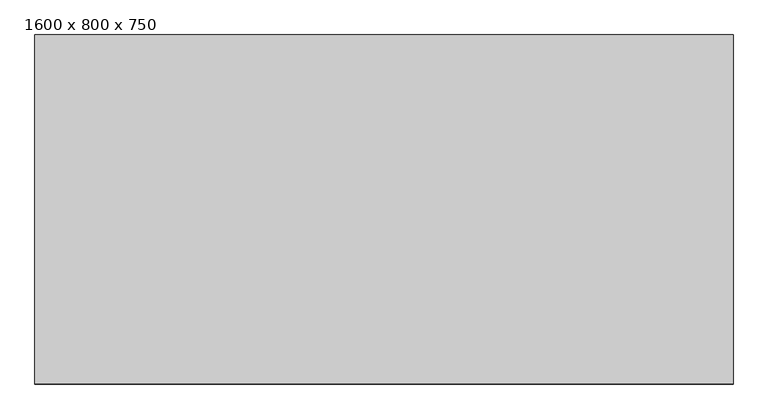
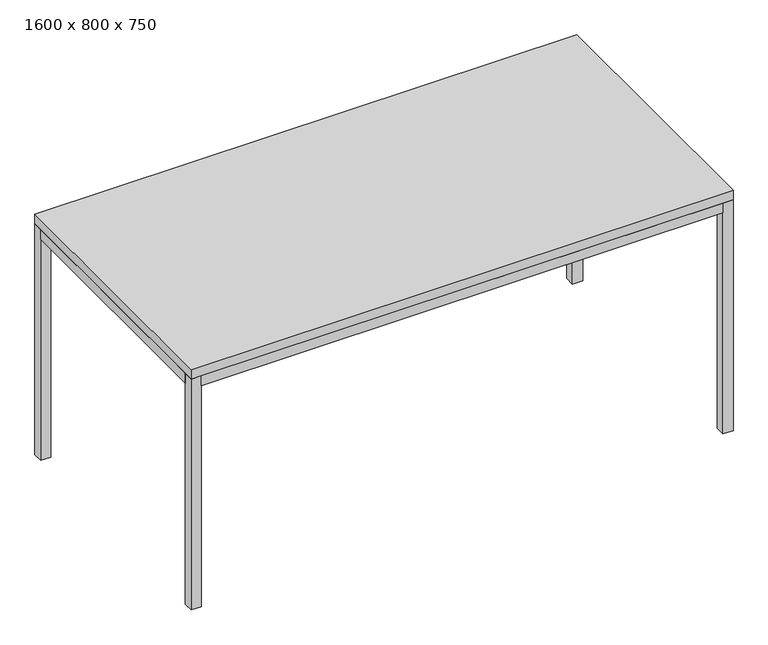
"""IFC4 building model written with IfcOpenShell, lengths in millimetres: furniture geometry, Bürotisch - Rechteckig : 1600 x 800 x 750."""

from ifc_helpers import new_model, si_unit, frame, origin, origin_with_axes, place, context, project, spatial, polyline, outline, extrude, source, transform, mapped, element, save


def furniture_1600_x_800_x_750_78cbd59d(model_context):
    return source(origin(), model_context, "Body", "SweptSolid", [
        extrude(outline(polyline([(-16.564671, 400.0), (-16.564671, 370.0), (-1556.564671, 370.0), (-1556.564671, 400.0), (-16.564671, 400.0)])), frame((0.0, 0.0, 690.0), z_axis=(0.0, 0.0, 1.0), x_axis=(1.0, 0.0, 0.0)), (0.0, 0.0, 1.0), 30.0),
        extrude(outline(polyline([(-16.564671, -400.0), (-1556.564671, -400.0), (-1556.564671, -370.0), (-16.564671, -370.0), (-16.564671, -400.0)])), frame((0.0, 0.0, 690.0), z_axis=(0.0, 0.0, 1.0), x_axis=(1.0, 0.0, 0.0)), (0.0, 0.0, 1.0), 30.0),
        extrude(outline(polyline([(-1556.564671, 370.0), (-1556.564671, -370.0), (-1586.564671, -370.0), (-1586.564671, 370.0), (-1556.564671, 370.0)])), frame((0.0, 0.0, 690.0), z_axis=(0.0, 0.0, 1.0), x_axis=(1.0, 0.0, 0.0)), (0.0, 0.0, 1.0), 30.0),
        extrude(outline(polyline([(-16.564671, 370.0), (13.435329, 370.0), (13.435329, -370.0), (-16.564671, -370.0), (-16.564671, 370.0)])), frame((0.0, 0.0, 690.0), z_axis=(0.0, 0.0, 1.0), x_axis=(1.0, 0.0, 0.0)), (0.0, 0.0, 1.0), 30.0),
        extrude(outline(polyline([(-1556.564671, 400.0), (-1556.564671, 370.0), (-1586.564671, 370.0), (-1586.564671, 400.0), (-1556.564671, 400.0)])), origin_with_axes(), (0.0, 0.0, 1.0), 720.0),
        extrude(outline(polyline([(-1556.564671, -400.0), (-1586.564671, -400.0), (-1586.564671, -370.0), (-1556.564671, -370.0), (-1556.564671, -400.0)])), origin_with_axes(), (0.0, 0.0, 1.0), 720.0),
        extrude(outline(polyline([(-16.564671, 400.0), (13.435329, 400.0), (13.435329, 370.0), (-16.564671, 370.0), (-16.564671, 400.0)])), origin_with_axes(), (0.0, 0.0, 1.0), 720.0),
        extrude(outline(polyline([(-16.564671, -400.0), (-16.564671, -370.0), (13.435329, -370.0), (13.435329, -400.0), (-16.564671, -400.0)])), origin_with_axes(), (0.0, 0.0, 1.0), 720.0),
        extrude(outline(polyline([(13.435329, 400.0), (13.435329, -400.0), (-1586.564671, -400.0), (-1586.564671, 400.0), (13.435329, 400.0)])), frame((0.0, 0.0, 720.0), z_axis=(0.0, 0.0, 1.0), x_axis=(1.0, 0.0, 0.0)), (0.0, 0.0, 1.0), 30.0),
    ])


if __name__ == "__main__":
    model = new_model("IFC4")
    model_context = context("Model", 3, world=origin())
    ifc_project = project(units=[si_unit("LENGTHUNIT", "METRE", prefix="MILLI")], contexts=[model_context])
    site = spatial("IfcSite", under=ifc_project)
    building = spatial("IfcBuilding", under=site)
    placement = place(None, origin())
    furniture_1600_x_800_x_750_shape = furniture_1600_x_800_x_750_78cbd59d(model_context)
    element("IfcFurniture", 1, ObjectType="Bürotisch - Rechteckig : 1600 x 800 x 750", at=placement, inside=building, context=model_context, shape_type="MappedRepresentation", body=[
        mapped(furniture_1600_x_800_x_750_shape, transform((0.0, 0.0, 0.0), x_axis=(1.0, 0.0, 0.0), y_axis=(0.0, 1.0, 0.0), z_axis=(0.0, 0.0, 1.0))),
    ])
    save(model, "model.ifc")

# Revit data of these elements
# Type "Bürotisch - Rechteckig : 1600 x 800 x 750"
#   Stärke Tischplatte = 0.030 m
#   Breite von Bein = 0.030 m
#   Höhe = 0.750 m
#   Länge = 1.600 m
#   Tiefe = 0.800 m
#   Im Vordergrund zeichnen [instance default] = yes
#   Bild = Metall - Aluminium
#   Tischplatte = Holz - BSH
#   Assembly Code = ""
# Element 1 (IfcFurniture, "Bürotisch - Rechteckig : 1600 x 800 x 750")
#   Materials on its faces: "Metall - Aluminium", "Holz - BSH"
# Materials
#   "Metall - Aluminium": class "Metall", colour RGB 247 247 247, transparency 0, Description = "Aluminium 6061", Cost = 0
#   "Holz - BSH": class "Holz", colour RGB 255 255 255, transparency 0, Cost = 0
